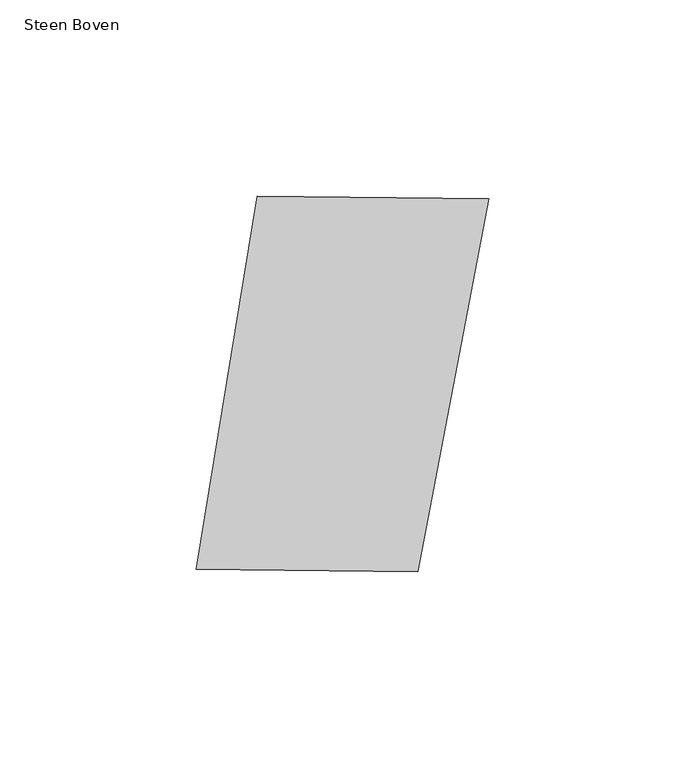
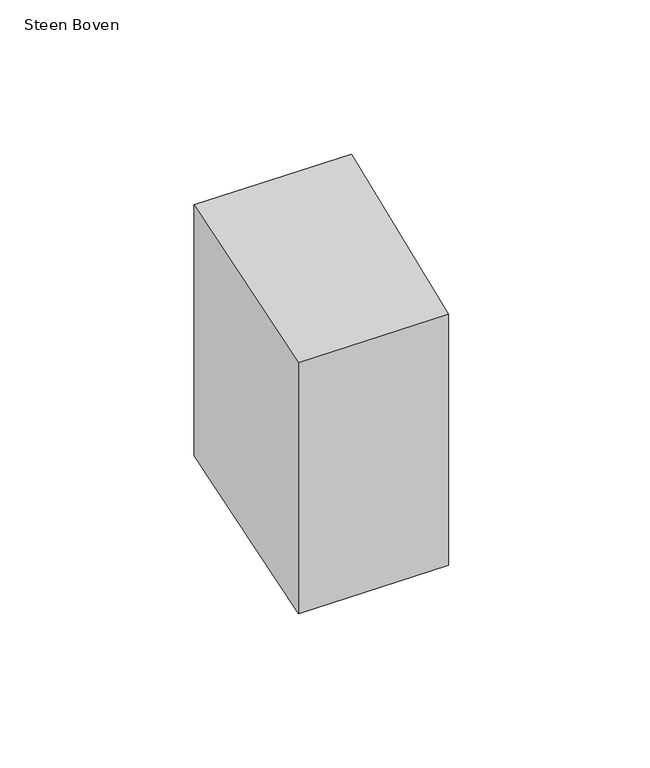
"""IFC4 building model written with IfcOpenShell, lengths in millimetres: proxy geometry, 00_GMA_steen_versie_4 : Steen Boven."""

from ifc_helpers import new_model, si_unit, origin, origin_with_axes, place, context, project, spatial, polyline, outline, extrude, source, transform, mapped, element, save


def steen_boven_6d657369(model_context):
    return source(origin(), model_context, "Body", "SweptSolid", [
        extrude(outline(polyline([(110.0512234, 118.5512029), (91.9904937, 23.66143), (35.6545533, 24.2803953), (51.0890541, 119.1795406), (110.0512234, 118.5512029)])), origin_with_axes(), (0.0, 0.0, 1.0), 100.0),
    ])


if __name__ == "__main__":
    model = new_model("IFC4")
    model_context = context("Model", 3, world=origin())
    ifc_project = project(units=[si_unit("LENGTHUNIT", "METRE", prefix="MILLI")], contexts=[model_context])
    site = spatial("IfcSite", under=ifc_project)
    building = spatial("IfcBuilding", under=site)
    placement = place(None, origin())
    steen_boven_shape = steen_boven_6d657369(model_context)
    element("IfcBuildingElementProxy", 1, Name="00_GMA_steen_versie_4 : Steen Boven", ObjectType="00_GMA_steen_versie_4 : Steen Boven", at=placement, inside=building, context=model_context, shape_type="MappedRepresentation", body=[
        mapped(steen_boven_shape, transform((0.0, 0.0, 0.0), x_axis=(1.0, 0.0, 0.0), y_axis=(0.0, 1.0, 0.0), z_axis=(0.0, 0.0, 1.0))),
    ])
    save(model, "model.ifc")

# Revit data of these elements
# Type "00_GMA_steen_versie_4 : Steen Boven"
#   StootVoegHalfBoven [instance default] = 5 mm
#   StootVoegHalf [instance default] = 5 mm
#   StootVoegBreedteOnder = 10 mm
#   StootVoegBreedteBoven = 10 mm
#   Steendikte = 100 mm
#   LintVoegOnderHalf = 5 mm
#   LintVoegOnder = 10 mm
#   LintVoegBovenHalf = 0 mm
#   LintVoegBoven = 0 mm
#   materiaal = none
#   MateriaalVoeg = none
#   Default Elevation = 0
